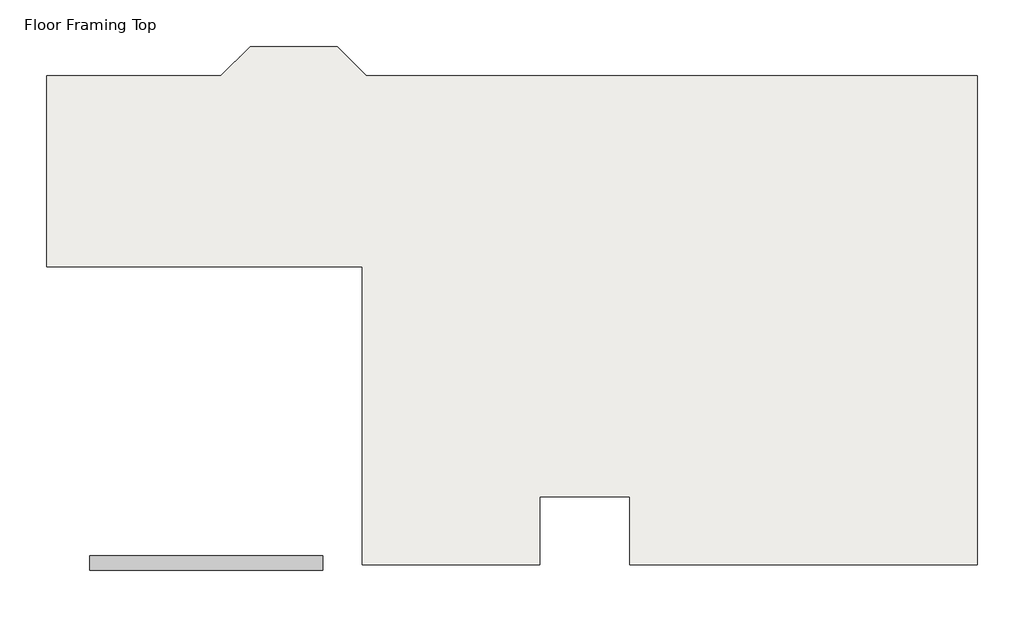
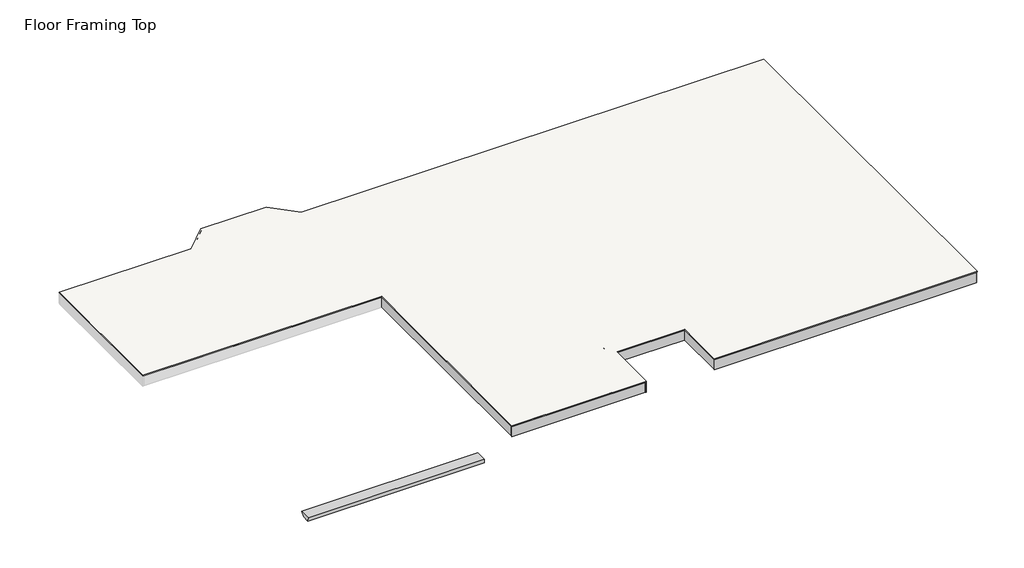
# One storey, part 1 of 4: 23 beams, 1 proxy, 1 slab.
"""IFC4 building model written with IfcOpenShell, lengths in millimetres."""

import ifcopenshell
import ifcopenshell.guid

model = None  # the IFC model being written
_history = None  # IfcOwnerHistory: only IFC2X3 demands one
_inside = {}  # id of a spatial element -> (the spatial element, [elements in it])
_under = {}  # id of a project, library or spatial element -> (it, [spatial elements below it])
_declared = {}  # id of a project -> (the project, [libraries it declares])
_typed = {}  # id of a type object -> (the type object, [elements of that type])
_made_of = {}  # id of a material, layer set ... -> (it, [elements and type objects made of it])


def new_model(schema):
    """Start an empty IFC model of exactly this schema.

    Asked for "IFC4X3", IfcOpenShell would pick the latest addendum, in which some entities
    have other attributes; the version numbers below select the first issue.
    IFC2X3 requires an IfcOwnerHistory on every rooted entity: one is made here for all.
    """
    global model, _history
    if schema == "IFC4X3":
        model = ifcopenshell.file(schema_version=(4, 3, 0, 0))
    else:
        model = ifcopenshell.file(schema=schema)
    _inside.clear()
    _under.clear()
    _declared.clear()
    _typed.clear()
    _made_of.clear()
    _history = None
    if model.schema == "IFC2X3":
        org = make("IfcOrganization", Name="unknown")
        user = make(
            "IfcPersonAndOrganization",
            ThePerson=make("IfcPerson", FamilyName="unknown"),
            TheOrganization=org,
        )
        app = make(
            "IfcApplication",
            ApplicationDeveloper=org,
            Version="unknown",
            ApplicationFullName="unknown",
            ApplicationIdentifier="unknown",
        )
        _history = make(
            "IfcOwnerHistory",
            OwningUser=user,
            OwningApplication=app,
            ChangeAction="ADDED",
            CreationDate=0,
        )
    return model


def make(cls, **values):
    """One entity of the class cls with the attributes given. An attribute that is None is left unset."""
    return model.create_entity(
        cls, **{name: value for name, value in values.items() if value is not None}
    )


def rooted(cls, **values):
    """An entity with a GlobalId (a new one), such as an element, a storey or a relation."""
    return make(cls, GlobalId=ifcopenshell.guid.new(), OwnerHistory=_history, **values)


def si_unit(unit_type, name, prefix=None):
    """IfcSIUnit, for example si_unit("LENGTHUNIT", "METRE", prefix="MILLI")."""
    return make("IfcSIUnit", UnitType=unit_type, Prefix=prefix, Name=name)


def assignment(units):
    """IfcUnitAssignment: the units of a project."""
    return None if units is None else make("IfcUnitAssignment", Units=units)


def point(xyz):
    """IfcCartesianPoint."""
    return None if xyz is None else make("IfcCartesianPoint", Coordinates=xyz)


def direction(xyz):
    """IfcDirection."""
    return None if xyz is None else make("IfcDirection", DirectionRatios=xyz)


def frame(location, z_axis=None, x_axis=None):
    """IfcAxis2Placement3D, a coordinate frame: its origin and axes. An axis left out is left unset."""
    return make(
        "IfcAxis2Placement3D",
        Location=point(location),
        Axis=direction(z_axis),
        RefDirection=direction(x_axis),
    )


def origin():
    """The frame at (0, 0, 0) with its axes left unset."""
    return frame((0.0, 0.0, 0.0))


def place(relative_to, where):
    """IfcLocalPlacement: puts the frame where relative to a parent placement (None: the world)."""
    return make(
        "IfcLocalPlacement", PlacementRelTo=relative_to, RelativePlacement=where
    )


def context(
    kind, dimensions, precision=None, world=None, true_north=None, identifier=None
):
    """IfcGeometricRepresentationContext, for example the 3D "Model" context."""
    return make(
        "IfcGeometricRepresentationContext",
        ContextIdentifier=identifier,
        ContextType=kind,
        CoordinateSpaceDimension=dimensions,
        Precision=precision,
        WorldCoordinateSystem=world,
        TrueNorth=true_north,
    )


def project(units=None, contexts=None):
    """IfcProject with its units and contexts."""
    return rooted(
        "IfcProject",
        Name="project",
        RepresentationContexts=contexts,
        UnitsInContext=assignment(units),
    )


def spatial(cls, under=None, at=None, **own):
    """A site, building, storey or space (cls), placed at a placement, below another one or the project."""
    s = rooted(cls, ObjectPlacement=at, **own)
    if under is not None:
        _under.setdefault(under.id(), (under, []))[1].append(s)
    return s


def polyline(points):
    """IfcPolyline through the points."""
    return make("IfcPolyline", Points=[point(p) for p in points])


def outline(outer, holes=None, kind="AREA"):
    """IfcArbitraryClosedProfileDef: a profile drawn as a closed curve; with holes, ...WithVoids."""
    if holes is None:
        return make("IfcArbitraryClosedProfileDef", ProfileType=kind, OuterCurve=outer)
    return make(
        "IfcArbitraryProfileDefWithVoids",
        ProfileType=kind,
        OuterCurve=outer,
        InnerCurves=holes,
    )


def extrude(swept, where, along, depth):
    """IfcExtrudedAreaSolid: the profile swept, set in the frame where, extruded along a direction by depth."""
    return make(
        "IfcExtrudedAreaSolid",
        SweptArea=swept,
        Position=where,
        ExtrudedDirection=direction(along),
        Depth=depth,
    )


def shape(context_of_items, identifier, shape_type, items):
    """IfcShapeRepresentation: the items that make up one representation, for example the "Body"."""
    return make(
        "IfcShapeRepresentation",
        ContextOfItems=context_of_items,
        RepresentationIdentifier=identifier,
        RepresentationType=shape_type,
        Items=items,
    )


def source(mapping_origin, context_of_items, identifier, shape_type, items):
    """IfcRepresentationMap: a shape defined once, which mapped items show again and again."""
    return make(
        "IfcRepresentationMap",
        MappingOrigin=mapping_origin,
        MappedRepresentation=shape(context_of_items, identifier, shape_type, items),
    )


def transform(
    local_origin,
    x_axis=None,
    y_axis=None,
    z_axis=None,
    scale=None,
    scale2=None,
    scale3=None,
    uniform=True,
):
    """IfcCartesianTransformationOperator3D, or its non-uniform kind. x_axis, y_axis, z_axis: its Axis1, 2, 3."""
    if uniform:
        return make(
            "IfcCartesianTransformationOperator3D",
            Axis1=direction(x_axis),
            Axis2=direction(y_axis),
            LocalOrigin=point(local_origin),
            Scale=scale,
            Axis3=direction(z_axis),
        )
    return make(
        "IfcCartesianTransformationOperator3DnonUniform",
        Axis1=direction(x_axis),
        Axis2=direction(y_axis),
        LocalOrigin=point(local_origin),
        Scale=scale,
        Axis3=direction(z_axis),
        Scale2=scale2,
        Scale3=scale3,
    )


def mapped(mapping_source, mapping_target):
    """IfcMappedItem: shows the shape of a source again, moved by a transform."""
    return make(
        "IfcMappedItem", MappingSource=mapping_source, MappingTarget=mapping_target
    )


def made_of(thing, what):
    """Note that an element or type object is made of a material, layer set ...; save() writes the relation."""
    if what is not None:
        _made_of.setdefault(what.id(), (what, []))[1].append(thing)
    return thing


def element(
    cls,
    number,
    at=None,
    inside=None,
    cuts=None,
    type_object=None,
    material=None,
    context=None,
    identifier="Body",
    shape_type=None,
    held_by="IfcProductDefinitionShape",
    body=None,
    shapes=None,
    **own,
):
    """One element of the class cls, such as IfcWall. Its Tag is "e" and its number.

    at: its placement. inside: the storey or other place that contains it. cuts: it is an
    opening in that element (IfcRelVoidsElement). A single representation is given by context,
    identifier, shape_type and body (its items); several are given by shapes. held_by: the class
    of the entity that holds the representations. save() writes the other relations.
    """
    e = rooted(cls, Tag="e%d" % number, ObjectPlacement=at, **own)
    if body is not None:
        shapes = [shape(context, identifier, shape_type, body)]
    if shapes is not None:
        e.Representation = make(held_by, Representations=shapes)
    if inside is not None:
        _inside.setdefault(inside.id(), (inside, []))[1].append(e)
    if cuts is not None:
        rooted(
            "IfcRelVoidsElement", RelatingBuildingElement=cuts, RelatedOpeningElement=e
        )
    if type_object is not None:
        _typed.setdefault(type_object.id(), (type_object, []))[1].append(e)
    return made_of(e, material)


def aggregate(whole, parts):
    """IfcRelAggregates: a whole, such as a stair, and the parts it consists of."""
    return rooted("IfcRelAggregates", RelatingObject=whole, RelatedObjects=parts)


def save(model, path):
    """Write the relations noted so far, then the file.

    IfcRelAggregates (storeys below a building ...), IfcRelContainedInSpatialStructure (elements
    in a storey), IfcRelDefinesByType, IfcRelAssociatesMaterial and IfcRelDeclares: one each for
    every whole, place, type object, material and project.
    """
    for whole, parts in _under.values():
        aggregate(whole, parts)
    for where, things in _inside.values():
        rooted(
            "IfcRelContainedInSpatialStructure",
            RelatedElements=things,
            RelatingStructure=where,
        )
    for kind, things in _typed.values():
        rooted("IfcRelDefinesByType", RelatedObjects=things, RelatingType=kind)
    for what, things in _made_of.values():
        rooted("IfcRelAssociatesMaterial", RelatedObjects=things, RelatingMaterial=what)
    for by, libraries in _declared.values():
        rooted("IfcRelDeclares", RelatingContext=by, RelatedDefinitions=libraries)
    model.write(path)


def lvl_laminated_veneer_lumber_rim_board_88c66cea(model_context):
    return source(origin(), model_context, "Body", "SweptSolid", [
        extrude(outline(polyline([(3108.325, 15.875), (3108.325, -15.875), (-3130.55, -15.875), (-3130.55, 15.875), (3108.325, 15.875)])), frame((0.0, 0.0, -150.8125), z_axis=(0.0, 0.0, 1.0), x_axis=(1.0, 0.0, 0.0)), (0.0, 0.0, 1.0), 301.625),
    ])


def lvl_laminated_veneer_lumber_rim_board_7eb16bd1(model_context):
    return source(origin(), model_context, "Body", "SweptSolid", [
        extrude(outline(polyline([(6406.35625, 15.875), (6406.35625, -15.875), (-840.58125, -15.875), (-840.58125, 15.875), (6406.35625, 15.875)])), frame((0.0, 0.0, -150.8125), z_axis=(0.0, 0.0, 1.0), x_axis=(1.0, 0.0, 0.0)), (0.0, 0.0, 1.0), 301.625),
    ])


def lvl_laminated_veneer_lumber_rim_board_f89b900f(model_context):
    return source(origin(), model_context, "Body", "SweptSolid", [
        extrude(outline(polyline([(695.325, 15.875), (695.325, -15.875), (-695.325, -15.875), (-695.325, 15.875), (695.325, 15.875)])), frame((0.0, 0.0, -150.8125), z_axis=(0.0, 0.0, 1.0), x_axis=(1.0, 0.0, 0.0)), (0.0, 0.0, 1.0), 301.625),
    ])


def lvl_laminated_veneer_lumber_rim_board_571f3e0e(model_context):
    return source(origin(), model_context, "Body", "SweptSolid", [
        extrude(outline(polyline([(971.55, 15.875), (971.55, -15.875), (-971.55, -15.875), (-971.55, 15.875), (971.55, 15.875)])), frame((0.0, 0.0, -150.8125), z_axis=(0.0, 0.0, 1.0), x_axis=(1.0, 0.0, 0.0)), (0.0, 0.0, 1.0), 301.625),
    ])


def lvl_laminated_veneer_lumber_rim_board_1d56c707(model_context):
    return source(origin(), model_context, "Body", "SweptSolid", [
        extrude(outline(polyline([(727.075, 15.875), (727.075, -15.875), (-695.325, -15.875), (-695.325, 15.875), (727.075, 15.875)])), frame((0.0, 0.0, -150.8125), z_axis=(0.0, 0.0, 1.0), x_axis=(1.0, 0.0, 0.0)), (0.0, 0.0, 1.0), 301.625),
    ])


def lvl_laminated_veneer_lumber_rim_board_585cc746(model_context):
    return source(origin(), model_context, "Body", "SweptSolid", [
        extrude(outline(polyline([(1858.9625, 15.875), (1858.9625, -15.875), (-1827.2125, -15.875), (-1827.2125, 15.875), (1858.9625, 15.875)])), frame((0.0, 0.0, -150.8125), z_axis=(0.0, 0.0, 1.0), x_axis=(1.0, 0.0, 0.0)), (0.0, 0.0, 1.0), 301.625),
    ])


model = new_model("IFC4")

# Units and contexts
model_context = context("Model", 3, world=origin())
ifc_project = project(units=[si_unit("LENGTHUNIT", "METRE", prefix="MILLI")], contexts=[model_context])

# Site, building, storey
site = spatial("IfcSite", under=ifc_project)
building = spatial("IfcBuilding", under=site)
storey = spatial("IfcBuildingStorey", under=building, Name="Floor Framing Top", Elevation=0.0)

# Beams
placement = place(None, origin())
lvl_laminated_veneer_lumber_rim_board_shape = lvl_laminated_veneer_lumber_rim_board_88c66cea(model_context)
element("IfcBeam", 1, ObjectType="LVL-Laminated Veneer Lumber : Rim Board", at=placement, inside=storey, context=model_context, shape_type="MappedRepresentation", body=[
    mapped(lvl_laminated_veneer_lumber_rim_board_shape, transform((383.7347749, -2609.4790947, -150.8125), x_axis=(0.0, -1.0, 0.0), y_axis=(1.0, 0.0, 0.0), z_axis=(0.0, 0.0, 1.0))),
])
lvl_laminated_veneer_lumber_rim_board_2_shape = lvl_laminated_veneer_lumber_rim_board_7eb16bd1(model_context)
element("IfcBeam", 2, ObjectType="LVL-Laminated Veneer Lumber : Rim Board", at=placement, inside=storey, context=model_context, shape_type="MappedRepresentation", body=[
    mapped(lvl_laminated_veneer_lumber_rim_board_2_shape, transform((6805.9660249, -5733.6790947, -150.8125), x_axis=(1.0, 0.0, 0.0), y_axis=(0.0, 1.0, 0.0), z_axis=(0.0, 0.0, 1.0))),
])
lvl_laminated_veneer_lumber_rim_board_3_shape = lvl_laminated_veneer_lumber_rim_board_f89b900f(model_context)
element("IfcBeam", 3, ObjectType="LVL-Laminated Veneer Lumber : Rim Board", at=placement, inside=storey, context=model_context, shape_type="MappedRepresentation", body=[
    mapped(lvl_laminated_veneer_lumber_rim_board_3_shape, transform((5981.2597749, -5022.4790947, -150.8125), x_axis=(0.0, 1.0, 0.0), y_axis=(-1.0, 0.0, 0.0), z_axis=(0.0, 0.0, 1.0))),
])
lvl_laminated_veneer_lumber_rim_board_4_shape = lvl_laminated_veneer_lumber_rim_board_571f3e0e(model_context)
element("IfcBeam", 4, ObjectType="LVL-Laminated Veneer Lumber : Rim Board", at=placement, inside=storey, context=model_context, shape_type="MappedRepresentation", body=[
    mapped(lvl_laminated_veneer_lumber_rim_board_4_shape, transform((5025.5847749, -4311.2790947, -150.8125), x_axis=(-1.0, 0.0, 0.0), y_axis=(0.0, -1.0, 0.0), z_axis=(0.0, 0.0, 1.0))),
])
lvl_laminated_veneer_lumber_rim_board_5_shape = lvl_laminated_veneer_lumber_rim_board_1d56c707(model_context)
element("IfcBeam", 5, ObjectType="LVL-Laminated Veneer Lumber : Rim Board", at=placement, inside=storey, context=model_context, shape_type="MappedRepresentation", body=[
    mapped(lvl_laminated_veneer_lumber_rim_board_5_shape, transform((4069.9097749, -5022.4790947, -150.8125), x_axis=(0.0, -1.0, 0.0), y_axis=(1.0, 0.0, 0.0), z_axis=(0.0, 0.0, 1.0))),
])
lvl_laminated_veneer_lumber_rim_board_6_shape = lvl_laminated_veneer_lumber_rim_board_585cc746(model_context)
element("IfcBeam", 6, ObjectType="LVL-Laminated Veneer Lumber : Rim Board", at=placement, inside=storey, context=model_context, shape_type="MappedRepresentation", body=[
    mapped(lvl_laminated_veneer_lumber_rim_board_6_shape, transform((2226.8222749, -5733.6790947, -150.8125), x_axis=(-1.0, 0.0, 0.0), y_axis=(0.0, -1.0, 0.0), z_axis=(0.0, 0.0, 1.0))),
])
element("IfcBeam", 7, ObjectType="Plywood Web Joist : 11 7/8 TJI 150", at=placement, inside=storey, context=model_context, shape_type="SweptSolid", body=[
    extrude(outline(polyline([(3912.7472749, -5717.8040947), (3903.2222749, -5717.8040947), (3903.2222749, 4456.4834053), (3912.7472749, 4456.4834053), (3912.7472749, -5717.8040947)])), frame((0.0, 0.0, -269.1410374), z_axis=(0.0, 0.0, 1.0), x_axis=(1.0, 0.0, 0.0)), (0.0, 0.0, 1.0), 237.3910374),
    extrude(outline(polyline([(3903.2222749, -663.2040947), (3903.2222749, 4456.4834053), (3912.7472749, 4456.4834053), (3912.7472749, -663.2040947), (3903.2222749, -663.2040947)])), frame((0.0, 0.0, -269.1410374), z_axis=(0.0, 0.0, 1.0), x_axis=(1.0, 0.0, 0.0)), (0.0, 0.0, 1.0), 237.3910374),
    extrude(outline(polyline([(0.0, 3888.9347749), (-38.1, 3888.9347749), (-38.1, 3903.2222749), (-31.75, 3903.2222749), (-31.75, 3912.7472749), (-38.1, 3912.7472749), (-38.1, 3927.0347749), (0.0, 3927.0347749), (0.0, 3888.9347749)])), frame((0.0, -5717.8040947, 0.0), z_axis=(0.0, 1.0, 0.0), x_axis=(0.0, 0.0, 1.0)), (0.0, 0.0, 1.0), 10174.2875),
    extrude(outline(polyline([(-263.525, 3927.0347749), (-263.525, 3912.7472749), (-269.1410374, 3912.7472749), (-269.1410374, 3903.2222749), (-263.525, 3903.2222749), (-263.525, 3888.9347749), (-301.625, 3888.9347749), (-301.625, 3927.0347749), (-263.525, 3927.0347749)])), frame((0.0, -5717.8040947, 0.0), z_axis=(0.0, 1.0, 0.0), x_axis=(0.0, 0.0, 1.0)), (0.0, 0.0, 1.0), 10174.2875),
    extrude(outline(polyline([(0.0, 3888.9347749), (-38.1, 3888.9347749), (-38.1, 3903.2222749), (-31.75, 3903.2222749), (-31.75, 3912.7472749), (-38.1, 3912.7472749), (-38.1, 3927.0347749), (0.0, 3927.0347749), (0.0, 3888.9347749)])), frame((0.0, -663.2040947, 0.0), z_axis=(0.0, 1.0, 0.0), x_axis=(0.0, 0.0, 1.0)), (0.0, 0.0, 1.0), 5119.6875),
    extrude(outline(polyline([(-263.525, 3927.0347749), (-263.525, 3912.7472749), (-269.1410374, 3912.7472749), (-269.1410374, 3903.2222749), (-263.525, 3903.2222749), (-263.525, 3888.9347749), (-301.625, 3888.9347749), (-301.625, 3927.0347749), (-263.525, 3927.0347749)])), frame((0.0, -663.2040947, 0.0), z_axis=(0.0, 1.0, 0.0), x_axis=(0.0, 0.0, 1.0)), (0.0, 0.0, 1.0), 5119.6875),
])
element("IfcBeam", 8, ObjectType="Plywood Web Joist : 11 7/8 TJI 150", at=placement, inside=storey, context=model_context, shape_type="SweptSolid", body=[
    extrude(outline(polyline([(3506.3472749, -5717.8040947), (3496.8222749, -5717.8040947), (3496.8222749, 4456.4834053), (3506.3472749, 4456.4834053), (3506.3472749, -5717.8040947)])), frame((0.0, 0.0, -269.1410374), z_axis=(0.0, 0.0, 1.0), x_axis=(1.0, 0.0, 0.0)), (0.0, 0.0, 1.0), 237.3910374),
    extrude(outline(polyline([(3496.8222749, -663.2040947), (3496.8222749, 4456.4834053), (3506.3472749, 4456.4834053), (3506.3472749, -663.2040947), (3496.8222749, -663.2040947)])), frame((0.0, 0.0, -269.1410374), z_axis=(0.0, 0.0, 1.0), x_axis=(1.0, 0.0, 0.0)), (0.0, 0.0, 1.0), 237.3910374),
    extrude(outline(polyline([(0.0, 3482.5347749), (-38.1, 3482.5347749), (-38.1, 3496.8222749), (-31.75, 3496.8222749), (-31.75, 3506.3472749), (-38.1, 3506.3472749), (-38.1, 3520.6347749), (0.0, 3520.6347749), (0.0, 3482.5347749)])), frame((0.0, -5717.8040947, 0.0), z_axis=(0.0, 1.0, 0.0), x_axis=(0.0, 0.0, 1.0)), (0.0, 0.0, 1.0), 10174.2875),
    extrude(outline(polyline([(-263.525, 3520.6347749), (-263.525, 3506.3472749), (-269.1410374, 3506.3472749), (-269.1410374, 3496.8222749), (-263.525, 3496.8222749), (-263.525, 3482.5347749), (-301.625, 3482.5347749), (-301.625, 3520.6347749), (-263.525, 3520.6347749)])), frame((0.0, -5717.8040947, 0.0), z_axis=(0.0, 1.0, 0.0), x_axis=(0.0, 0.0, 1.0)), (0.0, 0.0, 1.0), 10174.2875),
    extrude(outline(polyline([(0.0, 3482.5347749), (-38.1, 3482.5347749), (-38.1, 3496.8222749), (-31.75, 3496.8222749), (-31.75, 3506.3472749), (-38.1, 3506.3472749), (-38.1, 3520.6347749), (0.0, 3520.6347749), (0.0, 3482.5347749)])), frame((0.0, -663.2040947, 0.0), z_axis=(0.0, 1.0, 0.0), x_axis=(0.0, 0.0, 1.0)), (0.0, 0.0, 1.0), 5119.6875),
    extrude(outline(polyline([(-263.525, 3520.6347749), (-263.525, 3506.3472749), (-269.1410374, 3506.3472749), (-269.1410374, 3496.8222749), (-263.525, 3496.8222749), (-263.525, 3482.5347749), (-301.625, 3482.5347749), (-301.625, 3520.6347749), (-263.525, 3520.6347749)])), frame((0.0, -663.2040947, 0.0), z_axis=(0.0, 1.0, 0.0), x_axis=(0.0, 0.0, 1.0)), (0.0, 0.0, 1.0), 5119.6875),
])
element("IfcBeam", 9, ObjectType="Plywood Web Joist : 11 7/8 TJI 150", at=placement, inside=storey, context=model_context, shape_type="SweptSolid", body=[
    extrude(outline(polyline([(2693.5472749, -5717.8040947), (2684.0222749, -5717.8040947), (2684.0222749, 4456.4834053), (2693.5472749, 4456.4834053), (2693.5472749, -5717.8040947)])), frame((0.0, 0.0, -269.1410374), z_axis=(0.0, 0.0, 1.0), x_axis=(1.0, 0.0, 0.0)), (0.0, 0.0, 1.0), 237.3910374),
    extrude(outline(polyline([(2684.0222749, -663.2040947), (2684.0222749, 4456.4834053), (2693.5472749, 4456.4834053), (2693.5472749, -663.2040947), (2684.0222749, -663.2040947)])), frame((0.0, 0.0, -269.1410374), z_axis=(0.0, 0.0, 1.0), x_axis=(1.0, 0.0, 0.0)), (0.0, 0.0, 1.0), 237.3910374),
    extrude(outline(polyline([(0.0, 2669.7347749), (-38.1, 2669.7347749), (-38.1, 2684.0222749), (-31.75, 2684.0222749), (-31.75, 2693.5472749), (-38.1, 2693.5472749), (-38.1, 2707.8347749), (0.0, 2707.8347749), (0.0, 2669.7347749)])), frame((0.0, -5717.8040947, 0.0), z_axis=(0.0, 1.0, 0.0), x_axis=(0.0, 0.0, 1.0)), (0.0, 0.0, 1.0), 10174.2875),
    extrude(outline(polyline([(-263.525, 2707.8347749), (-263.525, 2693.5472749), (-269.1410374, 2693.5472749), (-269.1410374, 2684.0222749), (-263.525, 2684.0222749), (-263.525, 2669.7347749), (-301.625, 2669.7347749), (-301.625, 2707.8347749), (-263.525, 2707.8347749)])), frame((0.0, -5717.8040947, 0.0), z_axis=(0.0, 1.0, 0.0), x_axis=(0.0, 0.0, 1.0)), (0.0, 0.0, 1.0), 10174.2875),
    extrude(outline(polyline([(0.0, 2669.7347749), (-38.1, 2669.7347749), (-38.1, 2684.0222749), (-31.75, 2684.0222749), (-31.75, 2693.5472749), (-38.1, 2693.5472749), (-38.1, 2707.8347749), (0.0, 2707.8347749), (0.0, 2669.7347749)])), frame((0.0, -663.2040947, 0.0), z_axis=(0.0, 1.0, 0.0), x_axis=(0.0, 0.0, 1.0)), (0.0, 0.0, 1.0), 5119.6875),
    extrude(outline(polyline([(-263.525, 2707.8347749), (-263.525, 2693.5472749), (-269.1410374, 2693.5472749), (-269.1410374, 2684.0222749), (-263.525, 2684.0222749), (-263.525, 2669.7347749), (-301.625, 2669.7347749), (-301.625, 2707.8347749), (-263.525, 2707.8347749)])), frame((0.0, -663.2040947, 0.0), z_axis=(0.0, 1.0, 0.0), x_axis=(0.0, 0.0, 1.0)), (0.0, 0.0, 1.0), 5119.6875),
])
element("IfcBeam", 10, ObjectType="Plywood Web Joist : 11 7/8 TJI 150", at=placement, inside=storey, context=model_context, shape_type="SweptSolid", body=[
    extrude(outline(polyline([(2287.1472749, -5717.8040947), (2277.6222749, -5717.8040947), (2277.6222749, 4456.4834053), (2287.1472749, 4456.4834053), (2287.1472749, -5717.8040947)])), frame((0.0, 0.0, -269.1410374), z_axis=(0.0, 0.0, 1.0), x_axis=(1.0, 0.0, 0.0)), (0.0, 0.0, 1.0), 237.3910374),
    extrude(outline(polyline([(2277.6222749, -663.2040947), (2277.6222749, 4456.4834053), (2287.1472749, 4456.4834053), (2287.1472749, -663.2040947), (2277.6222749, -663.2040947)])), frame((0.0, 0.0, -269.1410374), z_axis=(0.0, 0.0, 1.0), x_axis=(1.0, 0.0, 0.0)), (0.0, 0.0, 1.0), 237.3910374),
    extrude(outline(polyline([(0.0, 2263.3347749), (-38.1, 2263.3347749), (-38.1, 2277.6222749), (-31.75, 2277.6222749), (-31.75, 2287.1472749), (-38.1, 2287.1472749), (-38.1, 2301.4347749), (0.0, 2301.4347749), (0.0, 2263.3347749)])), frame((0.0, -5717.8040947, 0.0), z_axis=(0.0, 1.0, 0.0), x_axis=(0.0, 0.0, 1.0)), (0.0, 0.0, 1.0), 10174.2875),
    extrude(outline(polyline([(-263.525, 2301.4347749), (-263.525, 2287.1472749), (-269.1410374, 2287.1472749), (-269.1410374, 2277.6222749), (-263.525, 2277.6222749), (-263.525, 2263.3347749), (-301.625, 2263.3347749), (-301.625, 2301.4347749), (-263.525, 2301.4347749)])), frame((0.0, -5717.8040947, 0.0), z_axis=(0.0, 1.0, 0.0), x_axis=(0.0, 0.0, 1.0)), (0.0, 0.0, 1.0), 10174.2875),
    extrude(outline(polyline([(0.0, 2263.3347749), (-38.1, 2263.3347749), (-38.1, 2277.6222749), (-31.75, 2277.6222749), (-31.75, 2287.1472749), (-38.1, 2287.1472749), (-38.1, 2301.4347749), (0.0, 2301.4347749), (0.0, 2263.3347749)])), frame((0.0, -663.2040947, 0.0), z_axis=(0.0, 1.0, 0.0), x_axis=(0.0, 0.0, 1.0)), (0.0, 0.0, 1.0), 5119.6875),
    extrude(outline(polyline([(-263.525, 2301.4347749), (-263.525, 2287.1472749), (-269.1410374, 2287.1472749), (-269.1410374, 2277.6222749), (-263.525, 2277.6222749), (-263.525, 2263.3347749), (-301.625, 2263.3347749), (-301.625, 2301.4347749), (-263.525, 2301.4347749)])), frame((0.0, -663.2040947, 0.0), z_axis=(0.0, 1.0, 0.0), x_axis=(0.0, 0.0, 1.0)), (0.0, 0.0, 1.0), 5119.6875),
])
element("IfcBeam", 11, ObjectType="Plywood Web Joist : 11 7/8 TJI 150", at=placement, inside=storey, context=model_context, shape_type="SweptSolid", body=[
    extrude(outline(polyline([(1880.7472749, -5717.8040947), (1871.2222749, -5717.8040947), (1871.2222749, 4456.4834053), (1880.7472749, 4456.4834053), (1880.7472749, -5717.8040947)])), frame((0.0, 0.0, -269.1410374), z_axis=(0.0, 0.0, 1.0), x_axis=(1.0, 0.0, 0.0)), (0.0, 0.0, 1.0), 237.3910374),
    extrude(outline(polyline([(1871.2222749, -663.2040947), (1871.2222749, 4456.4834053), (1880.7472749, 4456.4834053), (1880.7472749, -663.2040947), (1871.2222749, -663.2040947)])), frame((0.0, 0.0, -269.1410374), z_axis=(0.0, 0.0, 1.0), x_axis=(1.0, 0.0, 0.0)), (0.0, 0.0, 1.0), 237.3910374),
    extrude(outline(polyline([(0.0, 1856.9347749), (-38.1, 1856.9347749), (-38.1, 1871.2222749), (-31.75, 1871.2222749), (-31.75, 1880.7472749), (-38.1, 1880.7472749), (-38.1, 1895.0347749), (0.0, 1895.0347749), (0.0, 1856.9347749)])), frame((0.0, -5717.8040947, 0.0), z_axis=(0.0, 1.0, 0.0), x_axis=(0.0, 0.0, 1.0)), (0.0, 0.0, 1.0), 10174.2875),
    extrude(outline(polyline([(-263.525, 1895.0347749), (-263.525, 1880.7472749), (-269.1410374, 1880.7472749), (-269.1410374, 1871.2222749), (-263.525, 1871.2222749), (-263.525, 1856.9347749), (-301.625, 1856.9347749), (-301.625, 1895.0347749), (-263.525, 1895.0347749)])), frame((0.0, -5717.8040947, 0.0), z_axis=(0.0, 1.0, 0.0), x_axis=(0.0, 0.0, 1.0)), (0.0, 0.0, 1.0), 10174.2875),
    extrude(outline(polyline([(0.0, 1856.9347749), (-38.1, 1856.9347749), (-38.1, 1871.2222749), (-31.75, 1871.2222749), (-31.75, 1880.7472749), (-38.1, 1880.7472749), (-38.1, 1895.0347749), (0.0, 1895.0347749), (0.0, 1856.9347749)])), frame((0.0, -663.2040947, 0.0), z_axis=(0.0, 1.0, 0.0), x_axis=(0.0, 0.0, 1.0)), (0.0, 0.0, 1.0), 5119.6875),
    extrude(outline(polyline([(-263.525, 1895.0347749), (-263.525, 1880.7472749), (-269.1410374, 1880.7472749), (-269.1410374, 1871.2222749), (-263.525, 1871.2222749), (-263.525, 1856.9347749), (-301.625, 1856.9347749), (-301.625, 1895.0347749), (-263.525, 1895.0347749)])), frame((0.0, -663.2040947, 0.0), z_axis=(0.0, 1.0, 0.0), x_axis=(0.0, 0.0, 1.0)), (0.0, 0.0, 1.0), 5119.6875),
])
element("IfcBeam", 12, ObjectType="Plywood Web Joist : 11 7/8 TJI 150", at=placement, inside=storey, context=model_context, shape_type="SweptSolid", body=[
    extrude(outline(polyline([(1474.3472749, -5717.8040947), (1464.8222749, -5717.8040947), (1464.8222749, 4456.4834053), (1474.3472749, 4456.4834053), (1474.3472749, -5717.8040947)])), frame((0.0, 0.0, -269.1410374), z_axis=(0.0, 0.0, 1.0), x_axis=(1.0, 0.0, 0.0)), (0.0, 0.0, 1.0), 237.3910374),
    extrude(outline(polyline([(1464.8222749, -663.2040947), (1464.8222749, 4456.4834053), (1474.3472749, 4456.4834053), (1474.3472749, -663.2040947), (1464.8222749, -663.2040947)])), frame((0.0, 0.0, -269.1410374), z_axis=(0.0, 0.0, 1.0), x_axis=(1.0, 0.0, 0.0)), (0.0, 0.0, 1.0), 237.3910374),
    extrude(outline(polyline([(0.0, 1450.5347749), (-38.1, 1450.5347749), (-38.1, 1464.8222749), (-31.75, 1464.8222749), (-31.75, 1474.3472749), (-38.1, 1474.3472749), (-38.1, 1488.6347749), (0.0, 1488.6347749), (0.0, 1450.5347749)])), frame((0.0, -5717.8040947, 0.0), z_axis=(0.0, 1.0, 0.0), x_axis=(0.0, 0.0, 1.0)), (0.0, 0.0, 1.0), 10174.2875),
    extrude(outline(polyline([(-263.525, 1488.6347749), (-263.525, 1474.3472749), (-269.1410374, 1474.3472749), (-269.1410374, 1464.8222749), (-263.525, 1464.8222749), (-263.525, 1450.5347749), (-301.625, 1450.5347749), (-301.625, 1488.6347749), (-263.525, 1488.6347749)])), frame((0.0, -5717.8040947, 0.0), z_axis=(0.0, 1.0, 0.0), x_axis=(0.0, 0.0, 1.0)), (0.0, 0.0, 1.0), 10174.2875),
    extrude(outline(polyline([(0.0, 1450.5347749), (-38.1, 1450.5347749), (-38.1, 1464.8222749), (-31.75, 1464.8222749), (-31.75, 1474.3472749), (-38.1, 1474.3472749), (-38.1, 1488.6347749), (0.0, 1488.6347749), (0.0, 1450.5347749)])), frame((0.0, -663.2040947, 0.0), z_axis=(0.0, 1.0, 0.0), x_axis=(0.0, 0.0, 1.0)), (0.0, 0.0, 1.0), 5119.6875),
    extrude(outline(polyline([(-263.525, 1488.6347749), (-263.525, 1474.3472749), (-269.1410374, 1474.3472749), (-269.1410374, 1464.8222749), (-263.525, 1464.8222749), (-263.525, 1450.5347749), (-301.625, 1450.5347749), (-301.625, 1488.6347749), (-263.525, 1488.6347749)])), frame((0.0, -663.2040947, 0.0), z_axis=(0.0, 1.0, 0.0), x_axis=(0.0, 0.0, 1.0)), (0.0, 0.0, 1.0), 5119.6875),
])
element("IfcBeam", 13, ObjectType="Plywood Web Joist : 11 7/8 TJI 150", at=placement, inside=storey, context=model_context, shape_type="SweptSolid", body=[
    extrude(outline(polyline([(1067.9472749, -5717.8040947), (1058.4222749, -5717.8040947), (1058.4222749, 4456.4834053), (1067.9472749, 4456.4834053), (1067.9472749, -5717.8040947)])), frame((0.0, 0.0, -269.1410374), z_axis=(0.0, 0.0, 1.0), x_axis=(1.0, 0.0, 0.0)), (0.0, 0.0, 1.0), 237.3910374),
    extrude(outline(polyline([(1058.4222749, -663.2040947), (1058.4222749, 4456.4834053), (1067.9472749, 4456.4834053), (1067.9472749, -663.2040947), (1058.4222749, -663.2040947)])), frame((0.0, 0.0, -269.1410374), z_axis=(0.0, 0.0, 1.0), x_axis=(1.0, 0.0, 0.0)), (0.0, 0.0, 1.0), 237.3910374),
    extrude(outline(polyline([(0.0, 1044.1347749), (-38.1, 1044.1347749), (-38.1, 1058.4222749), (-31.75, 1058.4222749), (-31.75, 1067.9472749), (-38.1, 1067.9472749), (-38.1, 1082.2347749), (0.0, 1082.2347749), (0.0, 1044.1347749)])), frame((0.0, -5717.8040947, 0.0), z_axis=(0.0, 1.0, 0.0), x_axis=(0.0, 0.0, 1.0)), (0.0, 0.0, 1.0), 10174.2875),
    extrude(outline(polyline([(-263.525, 1082.2347749), (-263.525, 1067.9472749), (-269.1410374, 1067.9472749), (-269.1410374, 1058.4222749), (-263.525, 1058.4222749), (-263.525, 1044.1347749), (-301.625, 1044.1347749), (-301.625, 1082.2347749), (-263.525, 1082.2347749)])), frame((0.0, -5717.8040947, 0.0), z_axis=(0.0, 1.0, 0.0), x_axis=(0.0, 0.0, 1.0)), (0.0, 0.0, 1.0), 10174.2875),
    extrude(outline(polyline([(0.0, 1044.1347749), (-38.1, 1044.1347749), (-38.1, 1058.4222749), (-31.75, 1058.4222749), (-31.75, 1067.9472749), (-38.1, 1067.9472749), (-38.1, 1082.2347749), (0.0, 1082.2347749), (0.0, 1044.1347749)])), frame((0.0, -663.2040947, 0.0), z_axis=(0.0, 1.0, 0.0), x_axis=(0.0, 0.0, 1.0)), (0.0, 0.0, 1.0), 5119.6875),
    extrude(outline(polyline([(-263.525, 1082.2347749), (-263.525, 1067.9472749), (-269.1410374, 1067.9472749), (-269.1410374, 1058.4222749), (-263.525, 1058.4222749), (-263.525, 1044.1347749), (-301.625, 1044.1347749), (-301.625, 1082.2347749), (-263.525, 1082.2347749)])), frame((0.0, -663.2040947, 0.0), z_axis=(0.0, 1.0, 0.0), x_axis=(0.0, 0.0, 1.0)), (0.0, 0.0, 1.0), 5119.6875),
])
element("IfcBeam", 14, ObjectType="Plywood Web Joist : 11 7/8 TJI 150", at=placement, inside=storey, context=model_context, shape_type="SweptSolid", body=[
    extrude(outline(polyline([(661.5472749, -5717.8040947), (652.0222749, -5717.8040947), (652.0222749, 4456.4834053), (661.5472749, 4456.4834053), (661.5472749, -5717.8040947)])), frame((0.0, 0.0, -269.1410374), z_axis=(0.0, 0.0, 1.0), x_axis=(1.0, 0.0, 0.0)), (0.0, 0.0, 1.0), 237.3910374),
    extrude(outline(polyline([(652.0222749, -663.2040947), (652.0222749, 4456.4834053), (661.5472749, 4456.4834053), (661.5472749, -663.2040947), (652.0222749, -663.2040947)])), frame((0.0, 0.0, -269.1410374), z_axis=(0.0, 0.0, 1.0), x_axis=(1.0, 0.0, 0.0)), (0.0, 0.0, 1.0), 237.3910374),
    extrude(outline(polyline([(0.0, 637.7347749), (-38.1, 637.7347749), (-38.1, 652.0222749), (-31.75, 652.0222749), (-31.75, 661.5472749), (-38.1, 661.5472749), (-38.1, 675.8347749), (0.0, 675.8347749), (0.0, 637.7347749)])), frame((0.0, -5717.8040947, 0.0), z_axis=(0.0, 1.0, 0.0), x_axis=(0.0, 0.0, 1.0)), (0.0, 0.0, 1.0), 10174.2875),
    extrude(outline(polyline([(-263.525, 675.8347749), (-263.525, 661.5472749), (-269.1410374, 661.5472749), (-269.1410374, 652.0222749), (-263.525, 652.0222749), (-263.525, 637.7347749), (-301.625, 637.7347749), (-301.625, 675.8347749), (-263.525, 675.8347749)])), frame((0.0, -5717.8040947, 0.0), z_axis=(0.0, 1.0, 0.0), x_axis=(0.0, 0.0, 1.0)), (0.0, 0.0, 1.0), 10174.2875),
    extrude(outline(polyline([(0.0, 637.7347749), (-38.1, 637.7347749), (-38.1, 652.0222749), (-31.75, 652.0222749), (-31.75, 661.5472749), (-38.1, 661.5472749), (-38.1, 675.8347749), (0.0, 675.8347749), (0.0, 637.7347749)])), frame((0.0, -663.2040947, 0.0), z_axis=(0.0, 1.0, 0.0), x_axis=(0.0, 0.0, 1.0)), (0.0, 0.0, 1.0), 5119.6875),
    extrude(outline(polyline([(-263.525, 675.8347749), (-263.525, 661.5472749), (-269.1410374, 661.5472749), (-269.1410374, 652.0222749), (-263.525, 652.0222749), (-263.525, 637.7347749), (-301.625, 637.7347749), (-301.625, 675.8347749), (-263.525, 675.8347749)])), frame((0.0, -663.2040947, 0.0), z_axis=(0.0, 1.0, 0.0), x_axis=(0.0, 0.0, 1.0)), (0.0, 0.0, 1.0), 5119.6875),
])
element("IfcBeam", 15, ObjectType="Plywood Web Joist : 11 7/8 TJI 150", at=placement, inside=storey, context=model_context, shape_type="SweptSolid", body=[
    extrude(outline(polyline([(1474.3472749, -701.3040947), (1474.3472749, -5717.8040947), (1464.8222749, -5717.8040947), (1464.8222749, -701.3040947), (1474.3472749, -701.3040947)])), frame((0.0, 0.0, -269.1410374), z_axis=(0.0, 0.0, 1.0), x_axis=(1.0, 0.0, 0.0)), (0.0, 0.0, 1.0), 237.3910374),
    extrude(outline(polyline([(0.0, 1450.5347749), (-38.1, 1450.5347749), (-38.1, 1464.8222749), (-31.75, 1464.8222749), (-31.75, 1474.3472749), (-38.1, 1474.3472749), (-38.1, 1488.6347749), (0.0, 1488.6347749), (0.0, 1450.5347749)])), frame((0.0, -5717.8040947, 0.0), z_axis=(0.0, 1.0, 0.0), x_axis=(0.0, 0.0, 1.0)), (0.0, 0.0, 1.0), 5016.5),
    extrude(outline(polyline([(-263.525, 1488.6347749), (-263.525, 1474.3472749), (-269.1410374, 1474.3472749), (-269.1410374, 1464.8222749), (-263.525, 1464.8222749), (-263.525, 1450.5347749), (-301.625, 1450.5347749), (-301.625, 1488.6347749), (-263.525, 1488.6347749)])), frame((0.0, -5717.8040947, 0.0), z_axis=(0.0, 1.0, 0.0), x_axis=(0.0, 0.0, 1.0)), (0.0, 0.0, 1.0), 5016.5),
])
element("IfcBeam", 16, ObjectType="Plywood Web Joist : 11 7/8 TJI 150", at=placement, inside=storey, context=model_context, shape_type="SweptSolid", body=[
    extrude(outline(polyline([(1067.9472749, -701.3040947), (1067.9472749, -5717.8040947), (1058.4222749, -5717.8040947), (1058.4222749, -701.3040947), (1067.9472749, -701.3040947)])), frame((0.0, 0.0, -269.1410374), z_axis=(0.0, 0.0, 1.0), x_axis=(1.0, 0.0, 0.0)), (0.0, 0.0, 1.0), 237.3910374),
    extrude(outline(polyline([(0.0, 1044.1347749), (-38.1, 1044.1347749), (-38.1, 1058.4222749), (-31.75, 1058.4222749), (-31.75, 1067.9472749), (-38.1, 1067.9472749), (-38.1, 1082.2347749), (0.0, 1082.2347749), (0.0, 1044.1347749)])), frame((0.0, -5717.8040947, 0.0), z_axis=(0.0, 1.0, 0.0), x_axis=(0.0, 0.0, 1.0)), (0.0, 0.0, 1.0), 5016.5),
    extrude(outline(polyline([(-263.525, 1082.2347749), (-263.525, 1067.9472749), (-269.1410374, 1067.9472749), (-269.1410374, 1058.4222749), (-263.525, 1058.4222749), (-263.525, 1044.1347749), (-301.625, 1044.1347749), (-301.625, 1082.2347749), (-263.525, 1082.2347749)])), frame((0.0, -5717.8040947, 0.0), z_axis=(0.0, 1.0, 0.0), x_axis=(0.0, 0.0, 1.0)), (0.0, 0.0, 1.0), 5016.5),
])
element("IfcBeam", 17, ObjectType="Plywood Web Joist : 11 7/8 TJI 150", at=placement, inside=storey, context=model_context, shape_type="SweptSolid", body=[
    extrude(outline(polyline([(661.5472749, -701.3040947), (661.5472749, -5717.8040947), (652.0222749, -5717.8040947), (652.0222749, -701.3040947), (661.5472749, -701.3040947)])), frame((0.0, 0.0, -269.1410374), z_axis=(0.0, 0.0, 1.0), x_axis=(1.0, 0.0, 0.0)), (0.0, 0.0, 1.0), 237.3910374),
    extrude(outline(polyline([(0.0, 637.7347749), (-38.1, 637.7347749), (-38.1, 652.0222749), (-31.75, 652.0222749), (-31.75, 661.5472749), (-38.1, 661.5472749), (-38.1, 675.8347749), (0.0, 675.8347749), (0.0, 637.7347749)])), frame((0.0, -5717.8040947, 0.0), z_axis=(0.0, 1.0, 0.0), x_axis=(0.0, 0.0, 1.0)), (0.0, 0.0, 1.0), 5016.5),
    extrude(outline(polyline([(-263.525, 675.8347749), (-263.525, 661.5472749), (-269.1410374, 661.5472749), (-269.1410374, 652.0222749), (-263.525, 652.0222749), (-263.525, 637.7347749), (-301.625, 637.7347749), (-301.625, 675.8347749), (-263.525, 675.8347749)])), frame((0.0, -5717.8040947, 0.0), z_axis=(0.0, 1.0, 0.0), x_axis=(0.0, 0.0, 1.0)), (0.0, 0.0, 1.0), 5016.5),
])
element("IfcBeam", 18, ObjectType="Plywood Web Joist : 11 7/8 TJI 150", at=placement, inside=storey, context=model_context, shape_type="SweptSolid", body=[
    extrude(outline(polyline([(1880.7472749, -701.3040947), (1880.7472749, -5717.8040947), (1871.2222749, -5717.8040947), (1871.2222749, -701.3040947), (1880.7472749, -701.3040947)])), frame((0.0, 0.0, -269.1410374), z_axis=(0.0, 0.0, 1.0), x_axis=(1.0, 0.0, 0.0)), (0.0, 0.0, 1.0), 237.3910374),
    extrude(outline(polyline([(0.0, 1856.9347749), (-38.1, 1856.9347749), (-38.1, 1871.2222749), (-31.75, 1871.2222749), (-31.75, 1880.7472749), (-38.1, 1880.7472749), (-38.1, 1895.0347749), (0.0, 1895.0347749), (0.0, 1856.9347749)])), frame((0.0, -5717.8040947, 0.0), z_axis=(0.0, 1.0, 0.0), x_axis=(0.0, 0.0, 1.0)), (0.0, 0.0, 1.0), 5016.5),
    extrude(outline(polyline([(-263.525, 1895.0347749), (-263.525, 1880.7472749), (-269.1410374, 1880.7472749), (-269.1410374, 1871.2222749), (-263.525, 1871.2222749), (-263.525, 1856.9347749), (-301.625, 1856.9347749), (-301.625, 1895.0347749), (-263.525, 1895.0347749)])), frame((0.0, -5717.8040947, 0.0), z_axis=(0.0, 1.0, 0.0), x_axis=(0.0, 0.0, 1.0)), (0.0, 0.0, 1.0), 5016.5),
])
element("IfcBeam", 19, ObjectType="Plywood Web Joist : 11 7/8 TJI 150", at=placement, inside=storey, context=model_context, shape_type="SweptSolid", body=[
    extrude(outline(polyline([(2287.1472749, -701.3040947), (2287.1472749, -5717.8040947), (2277.6222749, -5717.8040947), (2277.6222749, -701.3040947), (2287.1472749, -701.3040947)])), frame((0.0, 0.0, -269.1410374), z_axis=(0.0, 0.0, 1.0), x_axis=(1.0, 0.0, 0.0)), (0.0, 0.0, 1.0), 237.3910374),
    extrude(outline(polyline([(0.0, 2263.3347749), (-38.1, 2263.3347749), (-38.1, 2277.6222749), (-31.75, 2277.6222749), (-31.75, 2287.1472749), (-38.1, 2287.1472749), (-38.1, 2301.4347749), (0.0, 2301.4347749), (0.0, 2263.3347749)])), frame((0.0, -5717.8040947, 0.0), z_axis=(0.0, 1.0, 0.0), x_axis=(0.0, 0.0, 1.0)), (0.0, 0.0, 1.0), 5016.5),
    extrude(outline(polyline([(-263.525, 2301.4347749), (-263.525, 2287.1472749), (-269.1410374, 2287.1472749), (-269.1410374, 2277.6222749), (-263.525, 2277.6222749), (-263.525, 2263.3347749), (-301.625, 2263.3347749), (-301.625, 2301.4347749), (-263.525, 2301.4347749)])), frame((0.0, -5717.8040947, 0.0), z_axis=(0.0, 1.0, 0.0), x_axis=(0.0, 0.0, 1.0)), (0.0, 0.0, 1.0), 5016.5),
])
element("IfcBeam", 20, ObjectType="Plywood Web Joist : 11 7/8 TJI 150", at=placement, inside=storey, context=model_context, shape_type="SweptSolid", body=[
    extrude(outline(polyline([(2693.5472749, -701.3040947), (2693.5472749, -5717.8040947), (2684.0222749, -5717.8040947), (2684.0222749, -701.3040947), (2693.5472749, -701.3040947)])), frame((0.0, 0.0, -269.1410374), z_axis=(0.0, 0.0, 1.0), x_axis=(1.0, 0.0, 0.0)), (0.0, 0.0, 1.0), 237.3910374),
    extrude(outline(polyline([(0.0, 2669.7347749), (-38.1, 2669.7347749), (-38.1, 2684.0222749), (-31.75, 2684.0222749), (-31.75, 2693.5472749), (-38.1, 2693.5472749), (-38.1, 2707.8347749), (0.0, 2707.8347749), (0.0, 2669.7347749)])), frame((0.0, -5717.8040947, 0.0), z_axis=(0.0, 1.0, 0.0), x_axis=(0.0, 0.0, 1.0)), (0.0, 0.0, 1.0), 5016.5),
    extrude(outline(polyline([(-263.525, 2707.8347749), (-263.525, 2693.5472749), (-269.1410374, 2693.5472749), (-269.1410374, 2684.0222749), (-263.525, 2684.0222749), (-263.525, 2669.7347749), (-301.625, 2669.7347749), (-301.625, 2707.8347749), (-263.525, 2707.8347749)])), frame((0.0, -5717.8040947, 0.0), z_axis=(0.0, 1.0, 0.0), x_axis=(0.0, 0.0, 1.0)), (0.0, 0.0, 1.0), 5016.5),
])
element("IfcBeam", 21, ObjectType="Plywood Web Joist : 11 7/8 TJI 150", at=placement, inside=storey, context=model_context, shape_type="SweptSolid", body=[
    extrude(outline(polyline([(3099.9472749, -701.3040947), (3099.9472749, -5717.8040947), (3090.4222749, -5717.8040947), (3090.4222749, -701.3040947), (3099.9472749, -701.3040947)])), frame((0.0, 0.0, -269.1410374), z_axis=(0.0, 0.0, 1.0), x_axis=(1.0, 0.0, 0.0)), (0.0, 0.0, 1.0), 237.3910374),
    extrude(outline(polyline([(0.0, 3076.1347749), (-38.1, 3076.1347749), (-38.1, 3090.4222749), (-31.75, 3090.4222749), (-31.75, 3099.9472749), (-38.1, 3099.9472749), (-38.1, 3114.2347749), (0.0, 3114.2347749), (0.0, 3076.1347749)])), frame((0.0, -5717.8040947, 0.0), z_axis=(0.0, 1.0, 0.0), x_axis=(0.0, 0.0, 1.0)), (0.0, 0.0, 1.0), 5016.5),
    extrude(outline(polyline([(-263.525, 3114.2347749), (-263.525, 3099.9472749), (-269.1410374, 3099.9472749), (-269.1410374, 3090.4222749), (-263.525, 3090.4222749), (-263.525, 3076.1347749), (-301.625, 3076.1347749), (-301.625, 3114.2347749), (-263.525, 3114.2347749)])), frame((0.0, -5717.8040947, 0.0), z_axis=(0.0, 1.0, 0.0), x_axis=(0.0, 0.0, 1.0)), (0.0, 0.0, 1.0), 5016.5),
])
element("IfcBeam", 22, ObjectType="Plywood Web Joist : 11 7/8 TJI 150", at=placement, inside=storey, context=model_context, shape_type="SweptSolid", body=[
    extrude(outline(polyline([(3506.3472749, -701.3040947), (3506.3472749, -5717.8040947), (3496.8222749, -5717.8040947), (3496.8222749, -701.3040947), (3506.3472749, -701.3040947)])), frame((0.0, 0.0, -269.1410374), z_axis=(0.0, 0.0, 1.0), x_axis=(1.0, 0.0, 0.0)), (0.0, 0.0, 1.0), 237.3910374),
    extrude(outline(polyline([(0.0, 3482.5347749), (-38.1, 3482.5347749), (-38.1, 3496.8222749), (-31.75, 3496.8222749), (-31.75, 3506.3472749), (-38.1, 3506.3472749), (-38.1, 3520.6347749), (0.0, 3520.6347749), (0.0, 3482.5347749)])), frame((0.0, -5717.8040947, 0.0), z_axis=(0.0, 1.0, 0.0), x_axis=(0.0, 0.0, 1.0)), (0.0, 0.0, 1.0), 5016.5),
    extrude(outline(polyline([(-263.525, 3520.6347749), (-263.525, 3506.3472749), (-269.1410374, 3506.3472749), (-269.1410374, 3496.8222749), (-263.525, 3496.8222749), (-263.525, 3482.5347749), (-301.625, 3482.5347749), (-301.625, 3520.6347749), (-263.525, 3520.6347749)])), frame((0.0, -5717.8040947, 0.0), z_axis=(0.0, 1.0, 0.0), x_axis=(0.0, 0.0, 1.0)), (0.0, 0.0, 1.0), 5016.5),
])
element("IfcBeam", 23, ObjectType="Plywood Web Joist : 11 7/8 TJI 150", at=placement, inside=storey, context=model_context, shape_type="SweptSolid", body=[
    extrude(outline(polyline([(3912.7472749, -701.3040947), (3912.7472749, -5717.8040947), (3903.2222749, -5717.8040947), (3903.2222749, -701.3040947), (3912.7472749, -701.3040947)])), frame((0.0, 0.0, -269.1410374), z_axis=(0.0, 0.0, 1.0), x_axis=(1.0, 0.0, 0.0)), (0.0, 0.0, 1.0), 237.3910374),
    extrude(outline(polyline([(0.0, 3888.9347749), (-38.1, 3888.9347749), (-38.1, 3903.2222749), (-31.75, 3903.2222749), (-31.75, 3912.7472749), (-38.1, 3912.7472749), (-38.1, 3927.0347749), (0.0, 3927.0347749), (0.0, 3888.9347749)])), frame((0.0, -5717.8040947, 0.0), z_axis=(0.0, 1.0, 0.0), x_axis=(0.0, 0.0, 1.0)), (0.0, 0.0, 1.0), 5016.5),
    extrude(outline(polyline([(-263.525, 3927.0347749), (-263.525, 3912.7472749), (-269.1410374, 3912.7472749), (-269.1410374, 3903.2222749), (-263.525, 3903.2222749), (-263.525, 3888.9347749), (-301.625, 3888.9347749), (-301.625, 3927.0347749), (-263.525, 3927.0347749)])), frame((0.0, -5717.8040947, 0.0), z_axis=(0.0, 1.0, 0.0), x_axis=(0.0, 0.0, 1.0)), (0.0, 0.0, 1.0), 5016.5),
])

# Proxy
element("IfcBuildingElementProxy", 24, Name="4\"x8\" Slab Edge", ObjectType="4\"x8\" Slab Edge", at=placement, inside=storey, context=model_context, shape_type="SweptSolid", body=[
    extrude(outline(polyline([(-5863.8540947, -606.191318), (-5559.115488, -600.0740006), (-5658.6559178, -703.692642), (-5861.8149889, -707.7708535), (-5863.8540947, -606.191318)])), frame((-5337.6152251, 0.0, 0.0), z_axis=(1.0, 0.0, 0.0), x_axis=(0.0, 1.0, 0.0)), (0.0, 0.0, 1.0), 4876.8),
])

# Slab
element("IfcSlab", 25, ObjectType="Structural Floor", at=placement, inside=storey, context=model_context, shape_type="SweptSolid", body=[
    extrude(outline(polyline([(-6240.9027251, 489.3209053), (-6240.9027251, 4488.2334053), (-2589.8122769, 4488.2334053), (-1980.2122769, 5097.8334053), (-160.6181733, 5097.8334053), (448.9818267, 4488.2334053), (13244.0722749, 4488.2334053), (13244.0722749, -5749.5540947), (5965.3847749, -5749.5540947), (5965.3847749, -4327.1540947), (4085.7847749, -4327.1540947), (4085.7847749, -5749.5540947), (367.8597749, -5749.5540947), (367.8597749, 489.3209053), (-6240.9027251, 489.3209053)])), frame((0.0, 0.0, -7.9375), z_axis=(0.0, 0.0, 1.0), x_axis=(1.0, 0.0, 0.0)), (0.0, 0.0, 1.0), 26.19375),
])

save(model, "model.ifc")

# Revit data of these elements
# Project information
#   Project Issue Date = "2022-10-14"
#   Project Status = "Project Status"
#   Client Name = "Team 6"
#   Project Address = "Enter address here"
#   Project Name = "JOHNSON RESIDENCE"
#   Project Number = "01"
# Grids (mm)
#   "1": line (-6252.015, 5673.323) -> (-6252.015, -7042.012)
#   "2": line (13255.185, 5673.323) -> (13255.185, -7042.012)
#   "A": line (-7655.483, 4499.346) -> (14853.483, 4499.346)
#   "B": line (-7655.483, -5762.254) -> (14853.483, -5762.254)
#   "2'": line (13712.385, 7840.557) -> (13712.385, -11272.413)
#   "1'": line (-6709.215, 7840.557) -> (-6709.215, -11272.413)
# Type "LVL-Laminated Veneer Lumber : Rim Board"
#   Assembly Code = "B10"
#   Cost = 4.6
#   Length [instance default] = 5' - 0"
#   b = 0' - 1 1/4"
#   d = 0' - 11 7/8"
#   Structural Material [instance default] = Softwood, Lumber
# Type "Plywood Web Joist : 11 7/8 TJI 150"
#   Assembly Code = "B10"
#   Cost = 17.5
#   Length [instance default] = 5' - 0"
#   b = 0' - 1 1/2"
#   d = 0' - 11 7/8"
#   Structural Material [instance default] = Softwood, Lumber
# Type "Structural Floor"
#   Function = 0
#   Layers, outside or top first: 0' - 0 5/16" "23/32\" OSB" (function 4); 0' - 0 23/32" "23/32\" OSB" (function 1)
# Elements 1, 2, 3, 4, 5, 6 (IfcBeam, "LVL-Laminated Veneer Lumber : Rim Board")
#   Comments = ""
#   Structural Material = Douglas Fir #2
#   Phase Created = New Construction
#   Materials on its faces: "Douglas Fir #2"
# Elements 7, 8, 9, 10, 11, 12, 13, 14, 15, 16, 17, 18, 19, 20, 21, 22, 23 (IfcBeam, "Plywood Web Joist : 11 7/8 TJI 150")
#   Structural Material = Douglas Fir #2
#   Phase Created = New Construction
#   Materials on its faces: "Douglas Fir #2"
# Element 24 (IfcBuildingElementProxy, "4\"x8\" Slab Edge")
#   built-in parameter 1001817 = -0.0200713 (stored number, unit not read)
#   Phase Created = New Construction
#   Materials on its faces: "Default Floor"
# Element 25 (IfcSlab, "Structural Floor")
#   built-in parameter 1001955 = -1.5708 (stored number, unit not read)
#   Height Offset From Level = 0' - 0 23/32"
#   Phase Created = New Construction
#   Materials on its faces: "23/32\" OSB"
# Materials
#   "Softwood, Lumber": class "Wood", colour RGB 223 192 134, transparency 0, Description = "Pinus Echinata", Cost = 0
#   "23/32\" OSB": class "Wood", colour RGB 193 140 64, transparency 0.87, Description = "Plywood, sheathing grade", Cost = 0
#   "Douglas Fir #2": class "Wood", colour RGB 223 192 134, transparency 0, Description = "Pinus Echinata", Cost = 0
#   "Default Floor": class "Miscellaneous", colour RGB 127 127 127, transparency 0, Cost = 0
